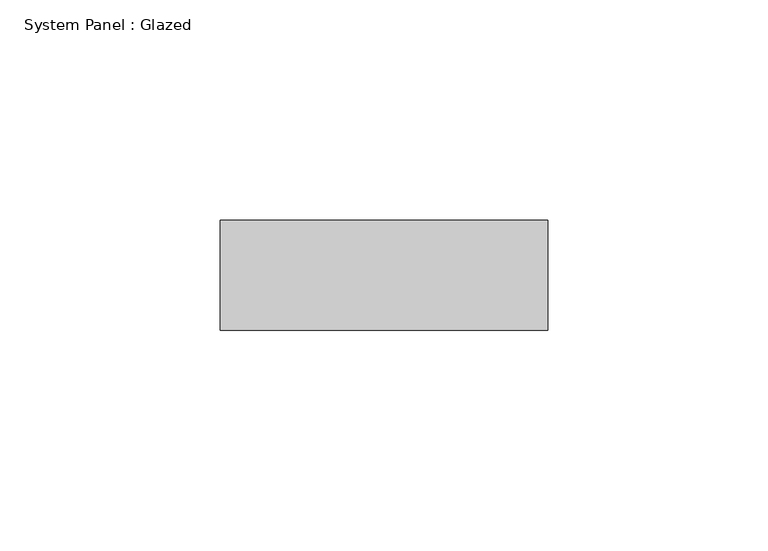
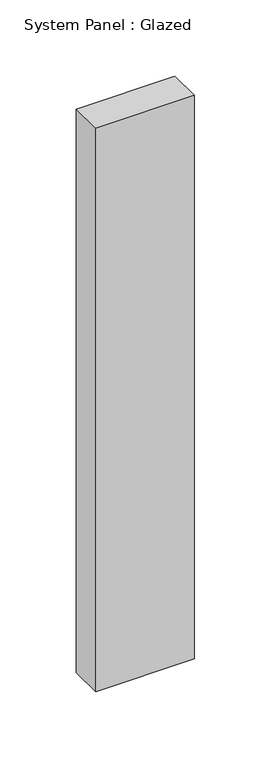
"""IFC4 building model written with IfcOpenShell, lengths in millimetres: plate geometry, System Panel : Glazed."""

from ifc_helpers import new_model, si_unit, origin, origin_with_axes, place, context, project, spatial, polyline, outline, extrude, source, transform, mapped, element, save


def system_panel_glazed_b42e89e7(model_context):
    return source(origin(), model_context, "Body", "SweptSolid", [
        extrude(outline(polyline([(37.2092572, 24.5), (-37.2092572, 24.5), (-37.2092572, 49.5), (37.2092572, 49.5), (37.2092572, 24.5)])), origin_with_axes(), (0.0, 0.0, 1.0), 450.0),
    ])


if __name__ == "__main__":
    model = new_model("IFC4")
    model_context = context("Model", 3, world=origin())
    ifc_project = project(units=[si_unit("LENGTHUNIT", "METRE", prefix="MILLI")], contexts=[model_context])
    site = spatial("IfcSite", under=ifc_project)
    building = spatial("IfcBuilding", under=site)
    placement = place(None, origin())
    system_panel_glazed_shape = system_panel_glazed_b42e89e7(model_context)
    element("IfcPlate", 1, ObjectType="System Panel : Glazed", at=placement, inside=building, context=model_context, shape_type="MappedRepresentation", body=[
        mapped(system_panel_glazed_shape, transform((0.0, 0.0, 0.0), x_axis=(1.0, 0.0, 0.0), y_axis=(0.0, 1.0, 0.0), z_axis=(0.0, 0.0, 1.0))),
    ])
    save(model, "model.ifc")

# Revit data of these elements
# Type "System Panel : Glazed"
#   Keynote = "H11"
#   Construction Type Id = "GSP4R"
#   Analytic Construction = "1/8 in Pilkington single glazing"
#   Visual Light Transmittance = 0.9
#   Solar Heat Gain Coefficient = 0.86
#   Heat Transfer Coefficient (U) = 6.7069 W/(m²·K)
# Element 1 (IfcPlate, "System Panel : Glazed")
#   Materials on its faces: "Glass"
# Materials
#   "Glass": class "Glass", colour RGB 0 128 192, transparency 0.9, Description = "Soda Lime Glass", Cost = 0
